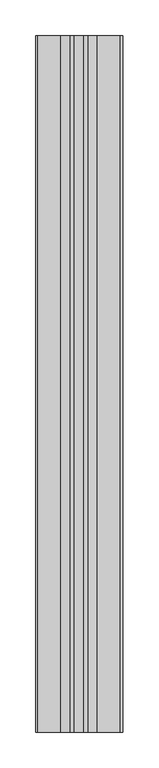
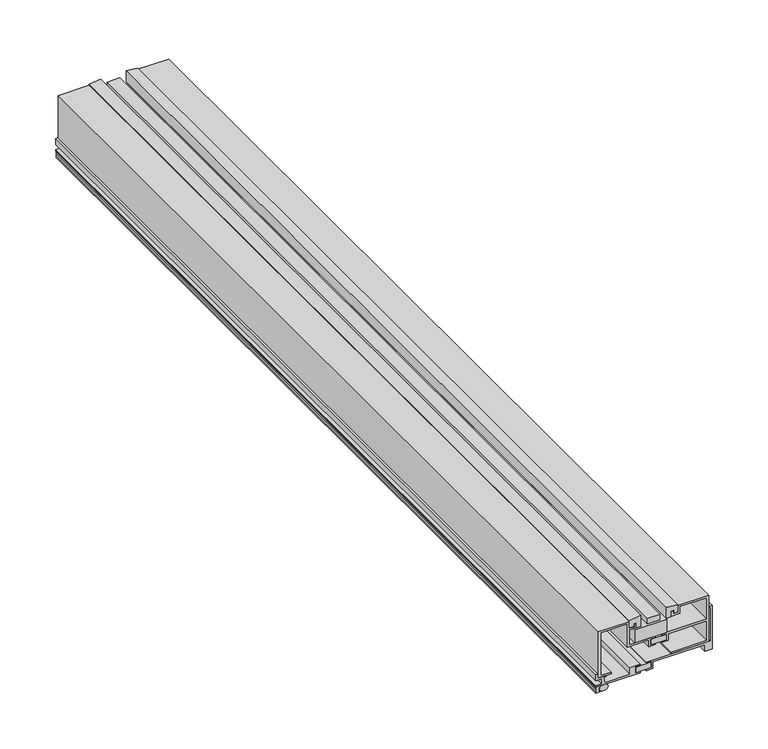
"""IFC4 building model written with IfcOpenShell, lengths in millimetres: proxy geometry, Generic Models 3:Generic Models 1:2:Generic Models 1:2 : Generic Models 3:Generic Models 1:300625:328150:Generic Models 1:2:Generic Models 1:2 : Generic Models 3:Generic Models 1:300625:328150 : Generic Models 3:Generic Models 1:2:Generic Models 1:2 : Generic Models 3:Generic Models 1:300625:328150:2 : Generic Models 3:Generic Models 1:2:Generic Models 1:2 : Generic Models 3:Generic Models 1:300625:328150:Generic Models 1:2:Generic Models 1:2 : Generic Models 3:Generic Models 1:300625:328150 : Generic Models 3:Generic Models 1:2:Generic Models 1:2 : Generic Models 3:Generic Models 1:300625:328150:300962."""

from ifc_helpers import new_model, si_unit, frame, origin, origin_with_axes, place, context, project, spatial, polyline, outline, extrude, source, transform, mapped, element, save


def generic_models_9e9fd1cb(model_context):
    return source(origin(), model_context, "Body", "SweptSolid", [
        extrude(outline(polyline([(560351.0390073, -573492.1001607), (560262.1390073, -573492.1001607), (560262.1390073, -572596.7501607), (560351.0390073, -572596.7501607), (560351.0390073, -573492.1001607)])), origin_with_axes(), (0.0, 0.0, 1.0), 6.35),
        extrude(outline(polyline([(5.3842368, 560365.833185), (6.35, 560366.2105936), (6.35, 560360.3425015), (5.4672112, 560361.9357182), (4.2258271, 560362.9099232), (2.8200508, 560363.1127111), (1.469803, 560362.5123576), (0.3863176, 560361.2027825), (0.0, 560360.3425015), (0.0, 560366.2105936), (0.9657632, 560365.833185), (3.175, 560365.5194989), (5.3842368, 560365.833185)])), frame((0.0, -573492.1001607, 0.0), z_axis=(0.0, 1.0, 0.0), x_axis=(0.0, 0.0, 1.0)), (0.0, 0.0, 1.0), 895.35),
        extrude(outline(polyline([(1.7974191, 560362.2697382), (3.175, 560362.7413739), (4.5525809, 560362.2697382), (5.657315, 560360.9482441), (6.2703961, 560359.0386299), (6.35, 560357.9788739), (6.2703961, 560356.919118), (5.657315, 560355.0095037), (4.5525809, 560353.6880097), (3.175, 560353.2163739), (1.7974191, 560353.6880097), (0.692685, 560355.0095037), (0.0796039, 560356.919118), (0.0, 560357.9788739), (0.0796039, 560359.0386299), (0.692685, 560360.9482441), (1.7974191, 560362.2697382)])), frame((0.0, -573492.1001607, 0.0), z_axis=(0.0, 1.0, 0.0), x_axis=(0.0, 0.0, 1.0)), (0.0, 0.0, 1.0), 895.35),
        extrude(outline(polyline([(0.0796039, 560254.666298), (0.692685, 560256.5759122), (1.7974191, 560257.8974063), (3.175, 560258.369042), (4.5525809, 560257.8974063), (5.657315, 560256.5759122), (6.2703961, 560254.666298), (6.35, 560253.606542), (6.2703961, 560252.5467861), (5.657315, 560250.6371719), (4.5525809, 560249.3156778), (3.175, 560248.844042), (1.7974191, 560249.3156778), (0.692685, 560250.6371719), (0.0796039, 560252.5467861), (0.0, 560253.606542), (0.0796039, 560254.666298)])), frame((0.0, -573566.7126607, 0.0), z_axis=(0.0, 1.0, 0.0), x_axis=(0.0, 0.0, 1.0)), (0.0, 0.0, 1.0), 969.9625),
        extrude(outline(polyline([(0.0, 560251.2429145), (0.3863176, 560250.3826335), (1.469803, 560249.0730583), (2.8200508, 560248.4727048), (4.2258271, 560248.6754927), (5.4672112, 560249.6496977), (6.35, 560251.2429145), (6.35, 560245.3748223), (5.3842368, 560245.752231), (3.175, 560246.065917), (0.9657632, 560245.752231), (0.0, 560245.3748223), (0.0, 560251.2429145)])), frame((0.0, -573566.7126607, 0.0), z_axis=(0.0, 1.0, 0.0), x_axis=(0.0, 0.0, 1.0)), (0.0, 0.0, 1.0), 969.9625),
        extrude(outline(polyline([(560319.1513516, -573566.7126607), (560285.8645165, -573566.7126607), (560285.8645165, -572596.7501607), (560319.1513516, -572596.7501607), (560319.1513516, -573566.7126607)])), frame((0.0, 0.0, 40.9290939), z_axis=(0.0, 0.0, 1.0), x_axis=(1.0, 0.0, 0.0)), (0.0, 0.0, 1.0), 14.2115027),
        extrude(outline(polyline([(560302.676817, -573566.7126607), (560286.5653808, -573566.7126607), (560286.5653808, -572596.7501607), (560302.676817, -572596.7501607), (560302.676817, -573566.7126607)])), frame((0.0, 0.0, 8.0979388), z_axis=(0.0, 0.0, 1.0), x_axis=(1.0, 0.0, 0.0)), (0.0, 0.0, 1.0), 6.0797872),
        extrude(outline(polyline([(53.9246391, 560363.1755343), (52.2575319, 560363.1755343), (52.2575319, 560364.4626548), (15.4696809, 560364.4626548), (15.4696809, 560297.8129872), (14.1777261, 560297.8129872), (14.1777261, 560302.676817), (8.0979388, 560302.676817), (8.0979388, 560297.8129872), (6.35, 560297.8129872), (6.35, 560304.3487585), (13.721742, 560304.3487585), (13.721742, 560358.318), (6.35, 560358.318), (6.35, 560366.2105936), (53.9246391, 560366.2105936), (53.9246391, 560363.1755343)])), frame((0.0, -573566.7126607, 0.0), z_axis=(0.0, 1.0, 0.0), x_axis=(0.0, 0.0, 1.0)), (0.0, 0.0, 1.0), 969.9625),
        extrude(outline(polyline([(8.0979388, 560280.7215688), (8.0979388, 560254.6773718), (13.9244136, 560253.7669851), (14.5730392, 560256.187689), (15.4696809, 560256.187689), (15.4696809, 560247.2416165), (20.2285817, 560247.2416165), (20.2285817, 560245.3748223), (13.721742, 560245.3748223), (13.721742, 560251.7585989), (8.0979388, 560251.7585989), (8.0979388, 560245.3748223), (6.35, 560245.3748223), (6.35, 560291.4292106), (8.0979388, 560291.4292106), (8.0979388, 560286.5653808), (14.1777261, 560286.5653808), (14.1777261, 560291.4292106), (15.4696809, 560291.4292106), (15.4696809, 560280.7215688), (8.0979388, 560280.7215688)])), frame((0.0, -573566.7126607, 0.0), z_axis=(0.0, 1.0, 0.0), x_axis=(0.0, 0.0, 1.0)), (0.0, 0.0, 1.0), 969.9625),
        extrude(outline(polyline([(560318.4673755, -573566.7126607), (560302.3559394, -573566.7126607), (560302.3559394, -572596.7501607), (560318.4673755, -572596.7501607), (560318.4673755, -573566.7126607)])), frame((0.0, 0.0, 32.9493731), z_axis=(0.0, 0.0, 1.0), x_axis=(1.0, 0.0, 0.0)), (0.0, 0.0, 1.0), 6.0797872),
        extrude(outline(polyline([(560311.6698356, -573566.7126607), (560298.9698356, -573566.7126607), (560298.9698356, -572596.7501607), (560311.6698356, -572596.7501607), (560311.6698356, -573566.7126607)])), frame((0.0, 0.0, 57.1165274), z_axis=(0.0, 0.0, 1.0), x_axis=(1.0, 0.0, 0.0)), (0.0, 0.0, 1.0), 6.3435484),
        extrude(outline(polyline([(62.433193, 560287.4773489), (56.7196524, 560287.4773489), (56.7196524, 560292.2314048), (68.7899095, 560292.2314048), (67.3290426, 560280.3335989), (59.4893332, 560280.3335989), (59.4893332, 560284.6316707), (62.433193, 560284.6316707), (62.433193, 560287.4773489)])), frame((0.0, -573566.7126607, 0.0), z_axis=(0.0, 1.0, 0.0), x_axis=(0.0, 0.0, 1.0)), (0.0, 0.0, 1.0), 969.9625),
        extrude(outline(polyline([(67.3290426, 560330.3060723), (68.7899095, 560318.4082665), (56.7196524, 560318.4082665), (56.7196524, 560323.1623223), (62.433193, 560323.1623223), (62.433193, 560326.0080005), (59.4893332, 560326.0080005), (59.4893332, 560330.3060723), (67.3290426, 560330.3060723)])), frame((0.0, -573566.7126607, 0.0), z_axis=(0.0, 1.0, 0.0), x_axis=(0.0, 0.0, 1.0)), (0.0, 0.0, 1.0), 969.9625),
        extrude(outline(polyline([(15.5459822, 560248.1867239), (15.5459822, 560261.273855), (17.4459157, 560261.273855), (17.4459157, 560250.6946362), (64.4122721, 560250.6946362), (64.4122721, 560278.0367904), (39.0291604, 560278.0367904), (39.0291604, 560300.4560058), (31.6574183, 560300.4560058), (31.6574183, 560307.2197691), (32.9493731, 560307.2197691), (32.9493731, 560302.3559394), (39.0291604, 560302.3559394), (39.0291604, 560307.2197691), (40.9290939, 560307.2197691), (40.9290939, 560279.9367239), (57.1165274, 560279.9367239), (57.1165274, 560287.0804739), (62.036318, 560287.0804739), (62.036318, 560285.0285457), (59.0924582, 560285.0285457), (59.0924582, 560279.9367239), (66.3122056, 560279.9367239), (66.3122056, 560248.1867239), (15.5459822, 560248.1867239)])), frame((0.0, -573566.7126607, 0.0), z_axis=(0.0, 1.0, 0.0), x_axis=(0.0, 0.0, 1.0)), (0.0, 0.0, 1.0), 969.9625),
        extrude(outline(polyline([(62.036318, 560325.6111255), (62.036318, 560323.5591973), (57.1165274, 560323.5591973), (57.1165274, 560332.6028808), (64.4024065, 560332.6028808), (64.4024065, 560360.5107931), (40.9290939, 560360.5107931), (40.9290939, 560313.6035457), (39.0291604, 560313.6035457), (39.0291604, 560318.4673755), (32.9493731, 560318.4673755), (32.9493731, 560313.6035457), (31.6574183, 560313.6035457), (31.6574183, 560320.367309), (39.0291604, 560320.367309), (39.0291604, 560360.5107931), (17.4681948, 560360.5107931), (17.4681948, 560323.5591973), (15.5459822, 560323.5591973), (15.5459822, 560362.4867239), (66.3122056, 560362.4867239), (66.3122056, 560330.7029473), (59.0924582, 560330.7029473), (59.0924582, 560325.6111255), (62.036318, 560325.6111255)])), frame((0.0, -573566.7126607, 0.0), z_axis=(0.0, 1.0, 0.0), x_axis=(0.0, 0.0, 1.0)), (0.0, 0.0, 1.0), 969.9625),
    ])


if __name__ == "__main__":
    model = new_model("IFC4")
    model_context = context("Model", 3, world=origin())
    ifc_project = project(units=[si_unit("LENGTHUNIT", "METRE", prefix="MILLI")], contexts=[model_context])
    site = spatial("IfcSite", under=ifc_project)
    building = spatial("IfcBuilding", under=site)
    placement = place(None, origin())
    generic_models_shape = generic_models_9e9fd1cb(model_context)
    element("IfcBuildingElementProxy", 1, Name="Generic Models 3:Generic Models 1:2:Generic Models 1:2 : Generic Models 3:Generic Models 1:300625:328150:Generic Models 1:2:Generic Models 1:2 : Generic Models 3:Generic Models 1:300625:328150 : Generic Models 3:Generic Models 1:2:Generic Models 1:2 : Generic Models 3:Generic Models 1:300625:328150:2 : Generic Models 3:Generic Models 1:2:Generic Models 1:2 : Generic Models 3:Generic Models 1:300625:328150:Generic Models 1:2:Generic Models 1:2 : Generic Models 3:Generic Models 1:300625:328150 : Generic Models 3:Generic Models 1:2:Generic Models 1:2 : Generic Models 3:Generic Models 1:300625:328150:300962", ObjectType="Generic Models 3:Generic Models 1:2:Generic Models 1:2 : Generic Models 3:Generic Models 1:300625:328150:Generic Models 1:2:Generic Models 1:2 : Generic Models 3:Generic Models 1:300625:328150 : Generic Models 3:Generic Models 1:2:Generic Models 1:2 : Generic Models 3:Generic Models 1:300625:328150:2 : Generic Models 3:Generic Models 1:2:Generic Models 1:2 : Generic Models 3:Generic Models 1:300625:328150:Generic Models 1:2:Generic Models 1:2 : Generic Models 3:Generic Models 1:300625:328150 : Generic Models 3:Generic Models 1:2:Generic Models 1:2 : Generic Models 3:Generic Models 1:300625:328150:300962", at=placement, inside=building, context=model_context, shape_type="MappedRepresentation", body=[
        mapped(generic_models_shape, transform((0.0, 0.0, 0.0), x_axis=(1.0, 0.0, 0.0), y_axis=(0.0, 1.0, 0.0), z_axis=(0.0, 0.0, 1.0))),
    ])
    save(model, "model.ifc")

# Revit data of these elements
# Type "Generic Models 3:Generic Models 1:2:Generic Models 1:2 : Generic Models 3:Generic Models 1:300625:328150:Generic Models 1:2:Generic Models 1:2 : Generic Models 3:Generic Models 1:300625:328150 : Generic Models 3:Generic Models 1:2:Generic Models 1:2 : Generic Models 3:Generic Models 1:300625:328150:2 : Generic Models 3:Generic Models 1:2:Generic Models 1:2 : Generic Models 3:Generic Models 1:300625:328150:Generic Models 1:2:Generic Models 1:2 : Generic Models 3:Generic Models 1:300625:328150 : Generic Models 3:Generic Models 1:2:Generic Models 1:2 : Generic Models 3:Generic Models 1:300625:328150:300962"
#   NameOverride = "Generic Models 3:Generic Models 1:2:Generic Models 1:2 : Generic Models 3:Generic Models 1:300625:328150:Generic Models 1:2:Generic Models 1:2 : Generic Models 3:Generic Models 1:300625:328150 : Generic Models 3:Generic Models 1:2:Generic Models 1:2 : Generic Models 3:Generic Models 1:300625:328150:300962"
#   ObjectTypeOverride = "Generic Models 1:2:Generic Models 1:2 : Generic Models 3:Generic Models 1:300625:328150 : Generic Models 3:Generic Models 1:2:Generic Models 1:2 : Generic Models 3:Generic Models 1:300625:328150"
#   Reference = "Generic Models 1"
#   Tag = "300962"
# Element 1 (IfcBuildingElementProxy, "Generic Models 3:Generic Models 1:2:Generic Models 1:2 : Generic Models 3:Generic Models 1:300625:328150:Generic Models 1:2:Generic Models 1:2 : Generic Models 3:Generic Models 1:300625:328150 : Generic Models 3:Generic Models 1:2:Generic Models 1:2 : Generic Models 3:Generic Models 1:300625:328150:2 : Generic Models 3:Generic Models 1:2:Generic Models 1:2 : Generic Models 3:Generic Models 1:300625:328150:Generic Models 1:2:Generic Models 1:2 : Generic Models 3:Generic Models 1:300625:328150 : Generic Models 3:Generic Models 1:2:Generic Models 1:2 : Generic Models 3:Generic Models 1:300625:328150:300962")
#   Materials on its faces: "THERMAL BROKEN ALUMINUM STOREFRONT", "SEALANT & BACKER ROD, IF NECESSARY"
# Materials
#   "THERMAL BROKEN ALUMINUM STOREFRONT": class "Unassigned", colour RGB 244 244 244, transparency 0, Cost = 0
#   "SEALANT & BACKER ROD, IF NECESSARY": class "Unassigned", colour RGB 120 120 120, transparency 0, Cost = 0
